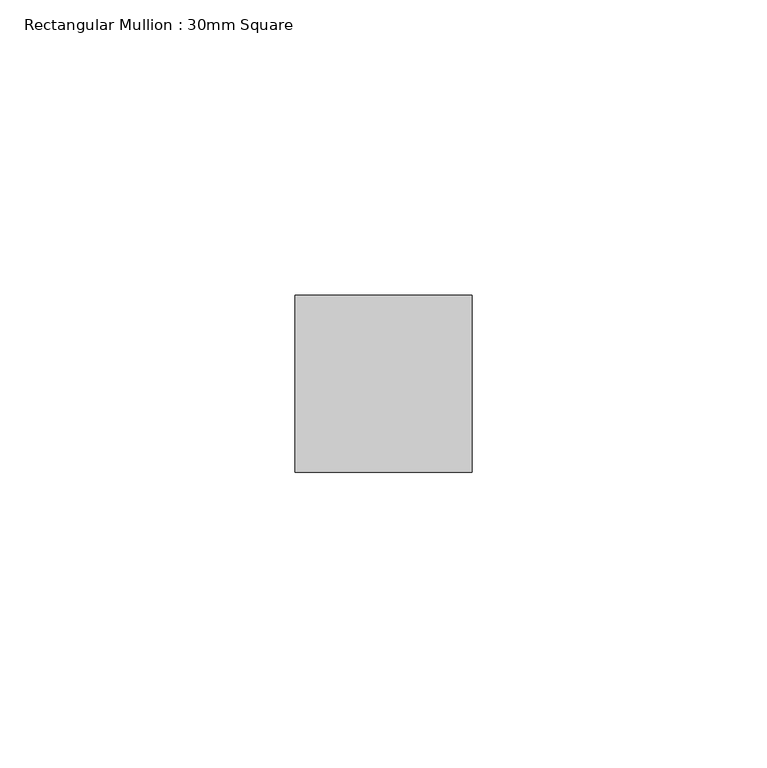
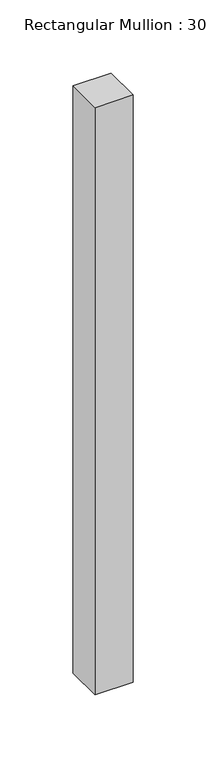
"""IFC4 building model written with IfcOpenShell, lengths in millimetres: member geometry, Rectangular Mullion : 30mm Square."""

from ifc_helpers import new_model, si_unit, frame, origin, place, context, project, spatial, polyline, outline, extrude, source, transform, mapped, element, save


def rectangular_mullion_30mm_square_f58054af(model_context):
    return source(origin(), model_context, "Body", "SweptSolid", [
        extrude(outline(polyline([(15.0, 15.0), (15.0, -15.0), (-15.0, -15.0), (-15.0, 15.0), (15.0, 15.0)])), frame((0.0, 0.0, -490.0541559), z_axis=(0.0, 0.0, 1.0), x_axis=(1.0, 0.0, 0.0)), (0.0, 0.0, 1.0), 490.0541559),
    ])


if __name__ == "__main__":
    model = new_model("IFC4")
    model_context = context("Model", 3, world=origin())
    ifc_project = project(units=[si_unit("LENGTHUNIT", "METRE", prefix="MILLI")], contexts=[model_context])
    site = spatial("IfcSite", under=ifc_project)
    building = spatial("IfcBuilding", under=site)
    placement = place(None, origin())
    rectangular_mullion_30mm_square_shape = rectangular_mullion_30mm_square_f58054af(model_context)
    element("IfcMember", 1, ObjectType="Rectangular Mullion : 30mm Square", at=placement, inside=building, context=model_context, shape_type="MappedRepresentation", body=[
        mapped(rectangular_mullion_30mm_square_shape, transform((0.0, 0.0, 0.0), x_axis=(1.0, 0.0, 0.0), y_axis=(0.0, 1.0, 0.0), z_axis=(0.0, 0.0, 1.0))),
    ])
    save(model, "model.ifc")

# Revit data of these elements
# Type "Rectangular Mullion : 30mm Square"
#   built-in parameter 1007304 = 0.0984252 (stored number, unit not read)
#   built-in parameter 1007301 = 0.0492126 (stored number, unit not read)
#   built-in parameter 1007300 = 0.0492126 (stored number, unit not read)
# Element 1 (IfcMember, "Rectangular Mullion : 30mm Square")
#   Materials on its faces: "Aluminum"
# Materials
#   "Aluminum": class "Metal", colour RGB 244 244 244, transparency 0, Description = "Aluminum 6061", Cost = 0
